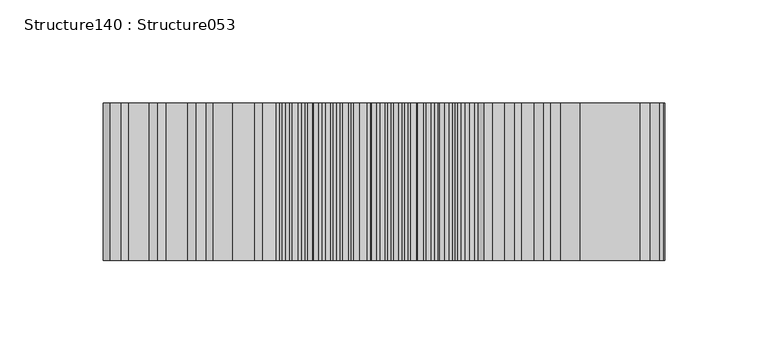
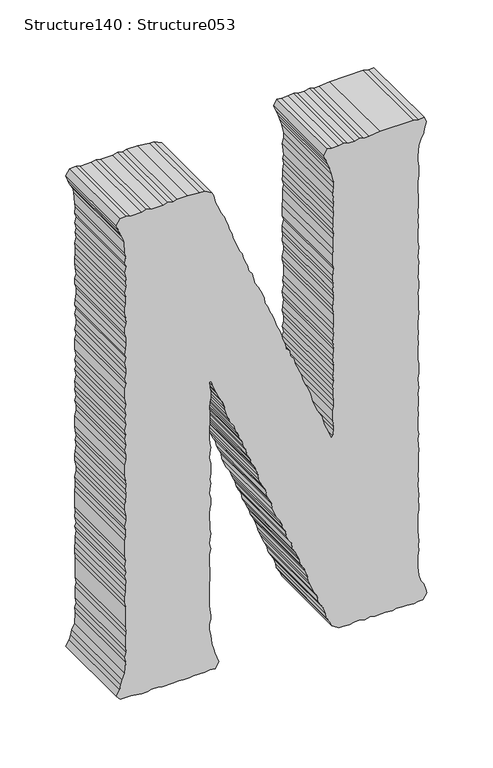
"""IFC4 building model written with IfcOpenShell, lengths in millimetres: proxy geometry, Structure140 : Structure053."""

from ifc_helpers import new_model, si_unit, frame, origin, place, context, project, spatial, polyline, outline, extrude, source, transform, mapped, element, save


def structure140_structure053_0c7b9da5(model_context):
    return source(origin(), model_context, "Body", "SweptSolid", [
        extrude(outline(polyline([(3575.0851816, -41553.7276732), (3583.2863152, -41554.8878023), (3589.1527492, -41556.0687912), (3593.8285667, -41556.0687912), (3597.9540049, -41554.8878023), (3602.0280957, -41554.8878023), (3607.3393366, -41555.489529), (3611.4134274, -41556.0687912), (3631.3410106, -41556.0687912), (3635.4407751, -41555.489529), (3644.8245022, -41555.489529), (3648.9258713, -41556.0687912), (3658.3015753, -41556.0687912), (3663.5598643, -41554.8878023), (3668.2437048, -41556.0687912), (3672.3691429, -41555.489529), (3677.0449605, -41554.8878023), (3681.7271964, -41555.489529), (3687.587212, -41555.489529), (3691.6869765, -41556.0687912), (3696.3884676, -41556.0687912), (3700.4705815, -41555.489529), (3704.5879966, -41554.8878023), (3709.8559132, -41554.8878023), (3714.5301261, -41556.0687912), (3718.6571688, -41555.489529), (3723.9154578, -41554.8878023), (3728.0152223, -41555.489529), (3732.7167134, -41554.8878023), (3742.6748889, -41554.8878023), (3747.3587295, -41556.0687912), (3752.6170184, -41555.489529), (3757.3185096, -41554.8878023), (3760.818152, -41555.489529), (3766.684586, -41556.0687912), (3774.8857196, -41556.0687912), (3780.7441306, -41555.489529), (3790.1294623, -41555.489529), (3794.2292268, -41556.0687912), (3798.9050443, -41555.489529), (3803.0064134, -41554.8878023), (3808.8888934, -41554.8878023), (3812.9726119, -41555.489529), (3818.2309008, -41556.0687912), (3817.6741031, -41554.8878023), (3812.9726119, -41552.5466843), (3808.290376, -41550.8088977), (3804.7730829, -41549.0486465), (3800.6717138, -41547.8676576), (3795.960595, -41544.924813), (3790.7039107, -41543.1870263), (3787.2042683, -41542.0060374), (3782.5027771, -41540.847513), (3777.8285642, -41539.0631928), (3773.7015215, -41537.3029416), (3770.2018791, -41534.4066305), (3766.1021146, -41533.2256416), (3760.2437036, -41530.8620592), (3757.3185096, -41529.7259992), (3752.6170184, -41527.3640214), (3748.5429276, -41526.1830325), (3743.8414364, -41523.8419145), (3739.1592005, -41523.2626523), (3733.8736333, -41520.3438767), (3730.3563402, -41519.1628878), (3725.6741043, -41516.7993054), (3722.1568112, -41515.0390542), (3716.8985223, -41513.3012676), (3712.7971532, -41512.7220054), (3708.087639, -41510.9617542), (3703.4134261, -41508.5981718), (3700.4705815, -41506.8603851), (3694.6298211, -41505.6793962), (3691.0868544, -41503.9191451), (3686.4030139, -41501.5780271), (3681.7271964, -41500.9987649), (3672.9435914, -41497.4782626), (3668.8261762, -41494.535418), (3664.1423357, -41492.7751669), (3660.6250426, -41491.6391069), (3655.9428067, -41489.2771291), (3651.8590883, -41488.6978668), (3647.1575971, -41486.3342844), (3643.6579547, -41484.0172355), (3638.3563415, -41483.4155088), (3634.2822506, -41481.0759955), (3630.1824862, -41479.3141398), (3625.472972, -41476.9746264), (3621.3732075, -41476.3953642), (3616.69739, -41473.4541241), (3613.1720739, -41471.6922684), (3607.3393366, -41469.9320173), (3603.7963698, -41469.3752195), (3599.7126514, -41467.5925039), (3591.5131224, -41464.070397), (3586.8116312, -41461.7533482), (3581.5276686, -41460.5723592), (3577.4535778, -41458.2312413), (3573.3265351, -41455.8692635), (3568.0682461, -41454.1314768), (3563.9412034, -41453.5522146), (3559.2669905, -41450.6093699), (3555.1848766, -41448.8491188), (3551.0658569, -41442.9874986), (3551.0658569, -41438.8877341), (3550.4833855, -41433.6053761), (3551.6675836, -41428.9263494), (3551.6675836, -41425.4042425), (3550.4833855, -41420.144349), (3551.6675836, -41415.4653223), (3550.4833855, -41411.3414887), (3551.0658569, -41405.4798685), (3551.0658569, -41401.9818307), (3550.4833855, -41396.097746), (3551.6675836, -41392.5997082), (3551.0658569, -41387.3173502), (3551.0658569, -41383.2159811), (3550.4833855, -41377.37843), (3551.0658569, -41373.2545964), (3551.0658569, -41369.1548319), (3556.3417965, -41365.6327251), (3559.8671125, -41366.813714), (3565.7094775, -41368.5739651), (3569.2524442, -41370.9375475), (3575.0851816, -41372.6753342), (3583.2863152, -41373.8338586), (3593.2541183, -41373.8338586), (3598.5284533, -41372.6753342), (3602.0280957, -41373.2545964), (3607.3393366, -41372.6753342), (3611.4134274, -41373.2545964), (3616.69739, -41373.8338586), (3631.3410106, -41373.8338586), (3635.4407751, -41372.6753342), (3640.114988, -41372.6753342), (3644.2420307, -41373.2545964), (3650.1004418, -41372.6753342), (3653.6000842, -41373.2545964), (3659.4584952, -41373.8338586), (3662.9854159, -41373.2545964), (3668.2437048, -41373.8338586), (3672.3691429, -41373.2545964), (3687.0127636, -41373.2545964), (3691.0868544, -41372.6753342), (3695.786741, -41373.2545964), (3701.6547796, -41373.8338586), (3705.7545441, -41372.6753342), (3709.8559132, -41373.8338586), (3719.2316172, -41373.8338586), (3725.0996559, -41373.2545964), (3728.5992983, -41373.8338586), (3734.47536, -41373.2545964), (3739.1592005, -41373.2545964), (3743.8414364, -41373.8338586), (3748.5429276, -41372.6753342), (3752.04257, -41373.2545964), (3757.8753073, -41373.8338586), (3762.0023501, -41372.6753342), (3771.3860772, -41372.6753342), (3775.4874463, -41373.8338586), (3784.8438951, -41373.8338586), (3790.1294623, -41373.2545964), (3795.4037973, -41373.8338586), (3799.5051664, -41373.2545964), (3804.7730829, -41373.8338586), (3809.4729695, -41373.8338586), (3812.9726119, -41373.2545964), (3818.2309008, -41372.6753342), (3822.348316, -41373.2545964), (3832.3161191, -41373.2545964), (3836.9919366, -41373.8338586), (3841.0900965, -41372.6753342), (3846.9757858, -41372.6753342), (3850.4754282, -41373.8338586), (3855.7353217, -41373.2545964), (3859.8591552, -41373.2545964), (3865.1190488, -41372.6753342), (3869.8189354, -41373.8338586), (3879.1769888, -41372.6753342), (3883.8881076, -41373.8338586), (3893.246161, -41373.8338586), (3898.5301236, -41373.2545964), (3903.2059411, -41373.8338586), (3907.3313793, -41373.2545964), (3912.0071968, -41373.8338586), (3916.6653636, -41373.2545964), (3926.6492128, -41373.2545964), (3930.1745289, -41373.8338586), (3940.1166583, -41373.8338586), (3944.8165449, -41372.6753342), (3953.5937315, -41372.6753342), (3959.4617701, -41373.8338586), (3962.9774586, -41373.8338586), (3972.9372387, -41372.6753342), (3977.6194746, -41370.9375475), (3982.8793681, -41368.5739651), (3986.4046842, -41367.9947029), (3992.2614906, -41366.2344517), (3996.9645864, -41367.9947029), (3996.390138, -41372.6753342), (3997.5486624, -41377.37843), (3997.5486624, -41406.662462), (3996.390138, -41416.0445845), (3996.390138, -41420.7236112), (3997.5486624, -41424.2457181), (3996.390138, -41428.9263494), (3996.390138, -41434.786365), (3997.5486624, -41438.3084719), (3996.9645864, -41442.9874986), (3996.9645864, -41448.8491188), (3997.5486624, -41452.9504879), (3992.2614906, -41455.8692635), (3987.5792547, -41454.1314768), (3982.3225704, -41451.7919634), (3978.2035506, -41450.6093699), (3972.9372387, -41448.8491188), (3964.1343784, -41447.1113321), (3959.4617701, -41447.1113321), (3954.7506513, -41448.2473921), (3944.235678, -41447.1113321), (3940.718385, -41447.6681299), (3936.0345445, -41447.1113321), (3930.7329312, -41447.6681299), (3925.4746423, -41447.6681299), (3921.3748778, -41448.2473921), (3916.6653636, -41447.1113321), (3912.5896682, -41447.6681299), (3903.2059411, -41447.6681299), (3897.3475301, -41448.2473921), (3887.9621984, -41448.2473921), (3884.4609514, -41447.1113321), (3878.5784713, -41448.2473921), (3873.9203044, -41448.2473921), (3870.4030114, -41447.6681299), (3864.5446004, -41448.2473921), (3859.8591552, -41447.1113321), (3856.3161885, -41447.1113321), (3850.4754282, -41448.2473921), (3846.9757858, -41448.2473921), (3842.2758992, -41447.1113321), (3832.8921721, -41447.1113321), (3828.2163546, -41447.6681299), (3823.5341187, -41447.1113321), (3818.2309008, -41448.2473921), (3813.5743386, -41447.6681299), (3810.0474179, -41447.1113321), (3804.1890069, -41447.6681299), (3800.0876378, -41448.2473921), (3794.8309535, -41447.1113321), (3790.1294623, -41447.1113321), (3785.4456218, -41448.2473921), (3780.7441306, -41447.1113321), (3777.2444882, -41448.2473921), (3772.5606477, -41447.6681299), (3767.2590344, -41447.6681299), (3762.5848215, -41447.1113321), (3757.3185096, -41447.1113321), (3753.8012165, -41448.2473921), (3744.4158848, -41448.2473921), (3738.5574738, -41447.1113321), (3735.0578314, -41447.1113321), (3730.3563402, -41448.2473921), (3729.1737467, -41449.428381), (3733.2991849, -41451.1902368), (3739.1592005, -41453.5522146), (3743.2332913, -41455.2900012), (3752.04257, -41457.6295146), (3755.559863, -41459.993097), (3760.2437036, -41462.3101459), (3764.9435901, -41464.070397), (3768.4432325, -41465.8322528), (3773.11905, -41467.0132417), (3777.8285642, -41468.1942306), (3781.9299333, -41469.9320173), (3786.0280932, -41472.2715306), (3791.8865042, -41474.635113), (3795.4037973, -41475.2143753), (3799.5051664, -41476.9746264), (3803.5872802, -41478.7124131), (3808.290376, -41481.0759955), (3813.5743386, -41482.2569844), (3817.6741031, -41485.17576), (3822.348316, -41485.7550222), (3825.2911606, -41488.6978668), (3830.5574726, -41489.8563913), (3834.6588416, -41491.6391069), (3838.7586061, -41492.7751669), (3844.0345457, -41494.535418), (3848.7167816, -41496.8990004), (3851.6612309, -41498.0799893), (3857.5019912, -41499.817776), (3860.4432313, -41500.9987649), (3864.5446004, -41503.3398829), (3869.8189354, -41505.100134), (3874.5043805, -41507.4396474), (3879.1769888, -41508.0189096), (3883.2863809, -41509.7791607), (3890.905043, -41513.3012676), (3895.5888836, -41516.2200432), (3900.8648231, -41517.4010321), (3904.9645876, -41518.5836256), (3909.0627475, -41521.5024012), (3914.3499193, -41522.6609256), (3917.8479571, -41524.4211767), (3922.5494483, -41526.1830325), (3926.6492128, -41527.3640214), (3930.1745289, -41529.7259992), (3934.8503464, -41531.4637859), (3939.5325823, -41533.2256416), (3944.235678, -41535.565155), (3947.7337158, -41536.1668816), (3952.9920048, -41538.4839305), (3957.1190475, -41539.6649194), (3961.2204166, -41541.4267752), (3966.5043792, -41543.1870263), (3971.1785921, -41546.1058019), (3974.7055128, -41547.2867908), (3978.8036727, -41549.0486465), (3982.8793681, -41550.8088977), (3988.7634528, -41551.9898866), (3992.2614906, -41553.7276732), (3995.7803883, -41560.1685557), (3995.7803883, -41564.2699248), (3996.9645864, -41574.8105717), (3996.9645864, -41584.1926942), (3995.7803883, -41587.7148011), (3996.9645864, -41592.3954324), (3995.7803883, -41596.5176613), (3995.7803883, -41607.0374484), (3996.9645864, -41611.1596774), (3995.7803883, -41615.238582), (3995.7803883, -41625.2224312), (3996.9645864, -41628.720469), (3996.390138, -41634.002827), (3991.0788971, -41637.5024694), (3986.4046842, -41635.7406136), (3982.8793681, -41634.6045536), (3977.6194746, -41631.6633136), (3973.5197101, -41630.4823247), (3962.9774586, -41629.9030625), (3959.4617701, -41629.3013358), (3953.5937315, -41629.9030625), (3950.0940891, -41628.720469), (3944.8165449, -41629.9030625), (3940.1166583, -41628.720469), (3936.0345445, -41629.3013358), (3931.3346579, -41628.720469), (3926.6492128, -41629.9030625), (3921.9733953, -41629.3013358), (3916.0909152, -41629.3013358), (3912.5896682, -41629.9030625), (3907.3313793, -41629.9030625), (3902.6314927, -41629.3013358), (3897.3475301, -41628.720469), (3893.822214, -41629.9030625), (3888.5623205, -41629.9030625), (3884.4609514, -41628.720469), (3879.1769888, -41628.720469), (3873.9203044, -41629.3013358), (3869.2444869, -41629.9030625), (3865.7015202, -41628.720469), (3861.0192843, -41629.9030625), (3855.1769193, -41628.720469), (3851.0595042, -41628.720469), (3846.3772683, -41629.9030625), (3841.6741725, -41628.720469), (3837.6000817, -41629.9030625), (3828.2163546, -41629.9030625), (3822.348316, -41628.720469), (3818.2309008, -41629.9030625), (3812.9726119, -41628.720469), (3809.4729695, -41629.9030625), (3804.1890069, -41628.720469), (3798.9050443, -41629.9030625), (3794.2292268, -41629.3013358), (3790.7039107, -41629.9030625), (3784.8438951, -41628.720469), (3780.7441306, -41629.9030625), (3776.0618947, -41628.720469), (3771.3860772, -41628.720469), (3766.684586, -41629.9030625), (3757.3185096, -41629.9030625), (3752.04257, -41629.3013358), (3747.9428055, -41628.720469), (3743.8414364, -41629.3013358), (3739.1592005, -41628.720469), (3733.8736333, -41629.3013358), (3729.7738688, -41629.9030625), (3725.0996559, -41629.9030625), (3719.2316172, -41628.720469), (3715.7143242, -41628.720469), (3709.8559132, -41629.9030625), (3706.3289925, -41629.3013358), (3701.6547796, -41629.3013358), (3696.9709391, -41629.9030625), (3682.3289231, -41629.9030625), (3678.2018803, -41629.3013358), (3672.9435914, -41629.9030625), (3667.6853024, -41628.720469), (3664.1423357, -41629.9030625), (3659.4584952, -41628.720469), (3654.7842823, -41629.3013358), (3649.5003197, -41629.3013358), (3644.8245022, -41629.9030625), (3640.114988, -41629.9030625), (3635.4407751, -41629.3013358), (3616.69739, -41629.3013358), (3612.0135494, -41628.720469), (3607.8961343, -41629.3013358), (3597.9540049, -41629.3013358), (3593.2541183, -41628.720469), (3589.1527492, -41629.9030625), (3584.4689087, -41629.3013358), (3574.5107332, -41629.9030625), (3569.2524442, -41632.2425758), (3565.1254015, -41633.4235647), (3561.025637, -41634.6045536), (3555.7416744, -41637.5024694), (3551.6675836, -41634.002827), (3551.6675836, -41624.6207045), (3550.4833855, -41615.238582), (3550.4833855, -41610.5804151), (3551.6675836, -41607.0374484), (3551.6675836, -41601.1982926), (3550.4833855, -41597.0969236), (3550.4833855, -41588.2940633), (3551.0658569, -41583.0117053), (3550.4833855, -41578.9344053), (3550.4833855, -41573.6520473), (3551.0658569, -41570.131545), (3551.0658569, -41560.1685557), (3551.6675836, -41555.489529), (3551.0658569, -41550.8088977), (3556.3417965, -41547.8676576), (3565.7094775, -41551.3881599), (3569.2524442, -41551.9898866), (3575.0851816, -41553.7276732)])), frame((0.0, 247945.1599557, 0.0), z_axis=(0.0, 1.0, 0.0), x_axis=(0.0, 0.0, 1.0)), (0.0, 0.0, 1.0), 76.2),
    ])


if __name__ == "__main__":
    model = new_model("IFC4")
    model_context = context("Model", 3, world=origin())
    ifc_project = project(units=[si_unit("LENGTHUNIT", "METRE", prefix="MILLI")], contexts=[model_context])
    site = spatial("IfcSite", under=ifc_project)
    building = spatial("IfcBuilding", under=site)
    placement = place(None, origin())
    structure140_structure053_shape = structure140_structure053_0c7b9da5(model_context)
    element("IfcBuildingElementProxy", 1, Name="Structure140 : Structure053", ObjectType="Structure140 : Structure053", at=placement, inside=building, context=model_context, shape_type="MappedRepresentation", body=[
        mapped(structure140_structure053_shape, transform((0.0, 0.0, 0.0), x_axis=(1.0, 0.0, 0.0), y_axis=(0.0, 1.0, 0.0), z_axis=(0.0, 0.0, 1.0))),
    ])
    save(model, "model.ifc")

# Revit data of these elements
# Type "Structure140 : Structure053"
#   NameOverride = "Structure053"
# Element 1 (IfcBuildingElementProxy, "Structure140 : Structure053")
#   Materials on its faces: "BRUSHED ALUM. LETTERING"
# Materials
#   "BRUSHED ALUM. LETTERING": class "Unassigned", colour RGB 169 181 186, transparency 0, Cost = 0
